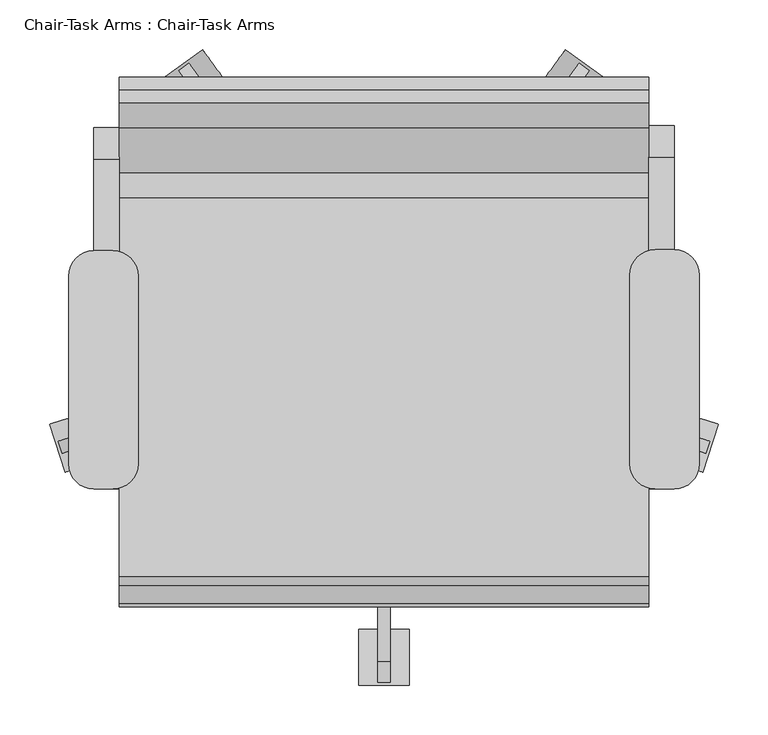
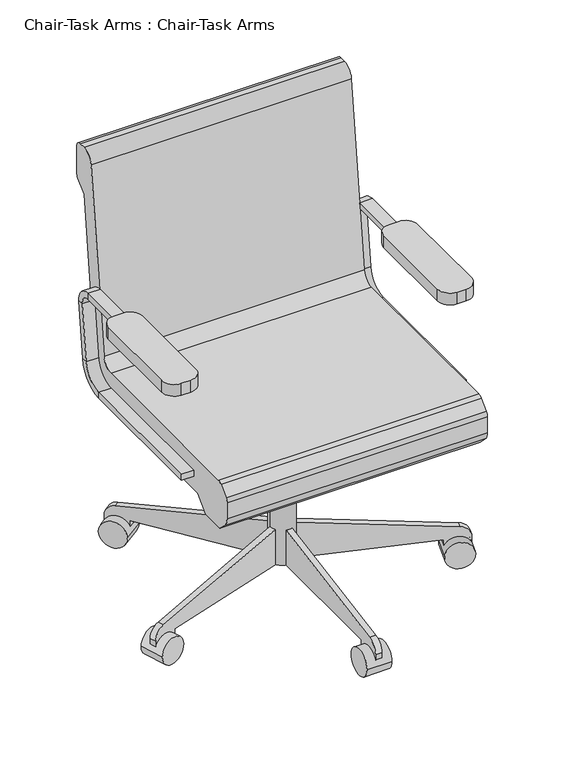
"""IFC4 building model written with IfcOpenShell, lengths in millimetres: furniture geometry, Chair-Task Arms : Chair-Task Arms."""

from ifc_helpers import new_model, si_unit, point, frame, frame_2d, origin, place, context, project, spatial, polyline, circle_curve, trimmed, segment, composite_curve, outline, extrude, source, transform, mapped, element, save
from ifc_brep_helpers import plane_surface, cylinder_surface, revolved_surface, advanced_brep


def chair_task_arms_chair_task_arms_3c69ee15(model_context):
    return source(origin(), model_context, "Body", "SolidModel", [
        extrude(outline(composite_curve([segment(trimmed(circle_curve(frame_2d((433.0908197, 48.8028048)), 25.4), [point((433.0908197, 74.2028048))], [point((458.4908197, 48.8028048))], False, "CARTESIAN"), True, "CONTINUOUS"), segment(polyline([(458.4908197, 48.8028048), (458.4908197, -141.6319091)]), True, "CONTINUOUS"), segment(trimmed(circle_curve(frame_2d((433.0908197, -141.6319091)), 25.4), [point((458.4908197, -141.6319091))], [point((433.0908197, -167.0319091))], False, "CARTESIAN"), True, "CONTINUOUS"), segment(polyline([(433.0908197, -167.0319091), (414.0408197, -167.0319091)]), True, "CONTINUOUS"), segment(trimmed(circle_curve(frame_2d((414.0408197, -141.6319091)), 25.4), [point((414.0408197, -167.0319091))], [point((388.6408197, -141.6319091))], False, "CARTESIAN"), True, "CONTINUOUS"), segment(polyline([(388.6408197, -141.6319091), (388.6408197, 48.8028048)]), True, "CONTINUOUS"), segment(trimmed(circle_curve(frame_2d((414.0408197, 48.8028048)), 25.4), [point((388.6408197, 48.8028048))], [point((414.0408197, 74.2028048))], False, "CARTESIAN"), True, "CONTINUOUS"), segment(polyline([(414.0408197, 74.2028048), (433.0908197, 74.2028048)]), True, "CONTINUOUS")], self_intersect=False)), frame((0.0, 0.0, 596.9), z_axis=(0.0, 0.0, 1.0), x_axis=(1.0, 0.0, 0.0)), (0.0, 0.0, 1.0), 25.4),
        extrude(outline(composite_curve([segment(trimmed(circle_curve(frame_2d((-132.0591803, 47.7575984)), 25.4), [point((-132.0591803, 73.1575984))], [point((-106.6591803, 47.7575984))], False, "CARTESIAN"), True, "CONTINUOUS"), segment(polyline([(-106.6591803, 47.7575984), (-106.6591803, -141.6319091)]), True, "CONTINUOUS"), segment(trimmed(circle_curve(frame_2d((-132.0591803, -141.6319091)), 25.4), [point((-106.6591803, -141.6319091))], [point((-132.0591803, -167.0319091))], False, "CARTESIAN"), True, "CONTINUOUS"), segment(polyline([(-132.0591803, -167.0319091), (-151.1091803, -167.0319091)]), True, "CONTINUOUS"), segment(trimmed(circle_curve(frame_2d((-151.1091803, -141.6319091)), 25.4), [point((-151.1091803, -167.0319091))], [point((-176.5091803, -141.6319091))], False, "CARTESIAN"), True, "CONTINUOUS"), segment(polyline([(-176.5091803, -141.6319091), (-176.5091803, 47.7575984)]), True, "CONTINUOUS"), segment(trimmed(circle_curve(frame_2d((-151.1091803, 47.7575984)), 25.4), [point((-176.5091803, 47.7575984))], [point((-151.1091803, 73.1575984))], False, "CARTESIAN"), True, "CONTINUOUS"), segment(polyline([(-151.1091803, 73.1575984), (-132.0591803, 73.1575984)]), True, "CONTINUOUS")], self_intersect=False)), frame((0.0, 0.0, 596.9), z_axis=(0.0, 0.0, 1.0), x_axis=(1.0, 0.0, 0.0)), (0.0, 0.0, 1.0), 25.4),
        advanced_brep(
        [(-151.1091803, -167.0319091, 412.75), (-125.7091803, -167.0319091, 412.75), (-125.7091803, -167.0319091, 425.45), (-151.1091803, -167.0319091, 425.45), (-151.1091803, 126.2388651, 425.45), (-151.1091803, 126.2388651, 412.75), (-125.7091803, 126.2388651, 425.45), (-125.7091803, 126.2388651, 412.75), (-151.1091803, 170.3844094, 464.7064065), (-151.1091803, 182.9974221, 463.2225227), (-125.7091803, 170.3844094, 464.7064065), (-125.7091803, 182.9974221, 463.2225227), (-151.1091803, 184.1806174, 581.9741742), (-151.1091803, 196.7936301, 580.4902904), (-125.7091803, 184.1806174, 581.9741742), (-125.7091803, 196.7936301, 580.4902904), (-151.1091803, 165.2610984, 603.25), (-151.1091803, 165.2610984, 615.95), (-125.7091803, 165.2610984, 603.25), (-125.7091803, 165.2610984, 615.95), (-151.1091803, -18.9459016, 615.95), (-151.1091803, -18.9459016, 603.25), (-125.7091803, -18.9459016, 603.25), (-125.7091803, -18.9459016, 615.95)],
        [
            (0, 1),
            (1, 2),
            (2, 3),
            (3, 0),
            (3, 4),
            (4, 5),
            (5, 0),
            (2, 6),
            (6, 4),
            (1, 7),
            (7, 6),
            (5, 7),
            (8, 9),
            (9, 5, circle_curve(frame((-151.1091803, 126.2388651, 469.9), z_axis=(-1.0, 0.0, 0.0), x_axis=(0.0, 0.0, -1.0)), 57.15)),
            (4, 8, circle_curve(frame((-151.1091803, 126.2388651, 469.9), z_axis=(1.0, 0.0, 0.0), x_axis=(0.0, 0.0, -1.0)), 44.45)),
            (10, 8),
            (6, 10, circle_curve(frame((-125.7091803, 126.2388651, 469.9), z_axis=(1.0, 0.0, 0.0), x_axis=(0.0, 0.0, -1.0)), 44.45)),
            (11, 10),
            (7, 11, circle_curve(frame((-125.7091803, 126.2388651, 469.9), z_axis=(1.0, 0.0, 0.0), x_axis=(0.0, 0.0, -1.0)), 57.15)),
            (9, 11),
            (8, 12),
            (12, 13),
            (13, 9),
            (10, 14),
            (14, 12),
            (11, 15),
            (15, 14),
            (13, 15),
            (16, 17),
            (17, 13, circle_curve(frame((-151.1091803, 165.2610984, 584.2), z_axis=(-1.0, 0.0, 0.0), x_axis=(0.0, 0.9931506043228768, -0.11684124756739202)), 31.75)),
            (12, 16, circle_curve(frame((-151.1091803, 165.2610984, 584.2), z_axis=(1.0, 0.0, 0.0), x_axis=(0.0, 0.9931506043228768, -0.11684124756739202)), 19.05)),
            (18, 16),
            (14, 18, circle_curve(frame((-125.7091803, 165.2610984, 584.2), z_axis=(1.0, 0.0, 0.0), x_axis=(0.0, 0.9931506043228768, -0.11684124756739202)), 19.05)),
            (19, 18),
            (15, 19, circle_curve(frame((-125.7091803, 165.2610984, 584.2), z_axis=(1.0, 0.0, 0.0), x_axis=(0.0, 0.9931506043228768, -0.11684124756739202)), 31.75)),
            (17, 19),
            (20, 21),
            (21, 22),
            (22, 23),
            (23, 20),
            (16, 21),
            (20, 17),
            (18, 22),
            (19, 23),
        ],
        [
            plane_surface(frame((-152.608212, -167.0319091, 419.1), z_axis=(0.0, -1.0, 0.0), x_axis=(0.0, 0.0, -1.0))),
            plane_surface(frame((-151.1091803, -167.0319091, 412.75), z_axis=(-1.0, 0.0, 0.0), x_axis=(0.0, 1.0, 0.0))),
            plane_surface(frame((-151.1091803, -167.0319091, 425.45), z_axis=(0.0, 0.0, 1.0), x_axis=(0.0, 1.0, 0.0))),
            plane_surface(frame((-125.7091803, -167.0319091, 425.45), z_axis=(1.0, 0.0, 0.0), x_axis=(0.0, 1.0, 0.0))),
            plane_surface(frame((-125.7091803, -167.0319091, 412.75), z_axis=(0.0, 0.0, -1.0), x_axis=(0.0, 1.0, 0.0))),
            plane_surface(frame((-151.1091803, 126.2388651, 469.9), z_axis=(-1.0, 0.0, 0.0), x_axis=(0.0, 0.0, -1.0))),
            revolved_surface(polyline([(-151.1091803, 126.2388651, 425.45), (-125.7091803, 126.2388651, 425.45)]), (-138.4091803, 126.2388651, 469.9), (-1.0, 0.0, 0.0)),
            plane_surface(frame((-125.7091803, 126.2388651, 469.9), z_axis=(1.0, 0.0, 0.0), x_axis=(0.0, 0.0, -1.0))),
            cylinder_surface(frame((-138.4091803, 126.2388651, 469.9), z_axis=(-1.0, 0.0, 0.0), x_axis=(0.0, 0.0, -1.0)), 57.15),
            plane_surface(frame((-151.1091803, 182.9974221, 463.2225227), z_axis=(-1.0, 0.0, 0.0), x_axis=(0.0, 0.1168412475673856, 0.9931506043228776))),
            plane_surface(frame((-151.1091803, 170.3844094, 464.7064065), z_axis=(0.0, -0.9931506043228776, 0.1168412475673856), x_axis=(0.0, 0.1168412475673856, 0.9931506043228776))),
            plane_surface(frame((-125.7091803, 170.3844094, 464.7064065), z_axis=(1.0, 0.0, 0.0), x_axis=(0.0, 0.1168412475673856, 0.9931506043228776))),
            plane_surface(frame((-125.7091803, 182.9974221, 463.2225227), z_axis=(0.0, 0.9931506043228776, -0.1168412475673856), x_axis=(0.0, 0.1168412475673856, 0.9931506043228776))),
            plane_surface(frame((-151.1091803, 165.2610984, 584.2), z_axis=(-1.0, 0.0, 0.0), x_axis=(0.0, 0.9931506043228768, -0.11684124756739202))),
            revolved_surface(polyline([(-151.1091803, 184.1806174123508, 581.9741742338413), (-125.7091803, 184.1806174123508, 581.9741742338413)]), (-138.4091803, 165.2610984, 584.2), (-1.0, 0.0, 0.0)),
            plane_surface(frame((-125.7091803, 165.2610984, 584.2), z_axis=(1.0, 0.0, 0.0), x_axis=(0.0, 0.9931506043228768, -0.11684124756739202))),
            cylinder_surface(frame((-138.4091803, 165.2610984, 584.2), z_axis=(-1.0, 0.0, 0.0), x_axis=(0.0, 0.9931506043228768, -0.11684124756739202)), 31.75),
            plane_surface(frame((-152.608212, -18.9459016, 609.6), z_axis=(0.0, -1.0, 0.0), x_axis=(0.0, 0.0, 1.0))),
            plane_surface(frame((-151.1091803, 165.2610984, 615.95), z_axis=(-1.0, 0.0, 0.0), x_axis=(0.0, -1.0, 0.0))),
            plane_surface(frame((-151.1091803, 165.2610984, 603.25), z_axis=(0.0, 0.0, -1.0), x_axis=(0.0, -1.0, 0.0))),
            plane_surface(frame((-125.7091803, 165.2610984, 603.25), z_axis=(1.0, 0.0, 0.0), x_axis=(0.0, -1.0, 0.0))),
            plane_surface(frame((-125.7091803, 165.2610984, 615.95), z_axis=(0.0, 0.0, 1.0), x_axis=(0.0, -1.0, 0.0))),
        ],
        [
            (0, [[1, 2, 3, 4]]),
            (1, [[5, 6, 7, -4]]),
            (2, [[8, 9, -5, -3]]),
            (3, [[10, 11, -8, -2]]),
            (4, [[-7, 12, -10, -1]]),
            (5, [[13, 14, -6, 15]]),
            (6, [[16, -15, -9, 17]]),
            (7, [[18, -17, -11, 19]]),
            (8, [[20, -19, -12, -14]]),
            (9, [[21, 22, 23, -13]]),
            (10, [[24, 25, -21, -16]]),
            (11, [[26, 27, -24, -18]]),
            (12, [[-23, 28, -26, -20]]),
            (13, [[29, 30, -22, 31]]),
            (14, [[32, -31, -25, 33]]),
            (15, [[34, -33, -27, 35]]),
            (16, [[36, -35, -28, -30]]),
            (17, [[37, 38, 39, 40]]),
            (18, [[41, -37, 42, -29]]),
            (19, [[43, -38, -41, -32]]),
            (20, [[44, -39, -43, -34]]),
            (21, [[-42, -40, -44, -36]]),
        ],
    ),
        advanced_brep(
        [(433.0908197, -167.0319091, 425.45), (407.6908197, -167.0319091, 425.45), (407.6908197, -167.0319091, 412.75), (433.0908197, -167.0319091, 412.75), (433.0908197, 128.329278, 412.75), (433.0908197, 128.329278, 425.45), (407.6908197, 128.329278, 412.75), (407.6908197, 128.329278, 425.45), (433.0908197, 185.0878351, 463.2225227), (433.0908197, 172.4748224, 464.7064065), (407.6908197, 185.0878351, 463.2225227), (407.6908197, 172.4748224, 464.7064065), (433.0908197, 198.884043, 580.4902904), (433.0908197, 186.2710303, 581.9741742), (407.6908197, 198.884043, 580.4902904), (407.6908197, 186.2710303, 581.9741742), (433.0908197, 167.3515113, 615.95), (433.0908197, 167.3515113, 603.25), (407.6908197, 167.3515113, 615.95), (407.6908197, 167.3515113, 603.25), (433.0908197, -18.9459016, 603.25), (433.0908197, -18.9459016, 615.95), (407.6908197, -18.9459016, 615.95), (407.6908197, -18.9459016, 603.25)],
        [
            (0, 1),
            (1, 2),
            (2, 3),
            (3, 0),
            (3, 4),
            (4, 5),
            (5, 0),
            (2, 6),
            (6, 4),
            (1, 7),
            (7, 6),
            (5, 7),
            (8, 9),
            (9, 5, circle_curve(frame((433.0908197, 128.329278, 469.9), z_axis=(-1.0, 0.0, 0.0), x_axis=(0.0, 0.0, -1.0)), 44.45)),
            (4, 8, circle_curve(frame((433.0908197, 128.329278, 469.9), z_axis=(1.0, 0.0, 0.0), x_axis=(0.0, 0.0, -1.0)), 57.15)),
            (10, 8),
            (6, 10, circle_curve(frame((407.6908197, 128.329278, 469.9), z_axis=(1.0, 0.0, 0.0), x_axis=(0.0, 0.0, -1.0)), 57.15)),
            (11, 10),
            (7, 11, circle_curve(frame((407.6908197, 128.329278, 469.9), z_axis=(1.0, 0.0, 0.0), x_axis=(0.0, 0.0, -1.0)), 44.45)),
            (9, 11),
            (8, 12),
            (12, 13),
            (13, 9),
            (10, 14),
            (14, 12),
            (11, 15),
            (15, 14),
            (13, 15),
            (16, 17),
            (17, 13, circle_curve(frame((433.0908197, 167.3515113, 584.2), z_axis=(-1.0, 0.0, 0.0), x_axis=(0.0, 0.9931506043228767, -0.1168412475673929)), 19.05)),
            (12, 16, circle_curve(frame((433.0908197, 167.3515113, 584.2), z_axis=(1.0, 0.0, 0.0), x_axis=(0.0, 0.9931506043228767, -0.1168412475673929)), 31.75)),
            (18, 16),
            (14, 18, circle_curve(frame((407.6908197, 167.3515113, 584.2), z_axis=(1.0, 0.0, 0.0), x_axis=(0.0, 0.9931506043228767, -0.1168412475673929)), 31.75)),
            (19, 18),
            (15, 19, circle_curve(frame((407.6908197, 167.3515113, 584.2), z_axis=(1.0, 0.0, 0.0), x_axis=(0.0, 0.9931506043228767, -0.1168412475673929)), 19.05)),
            (17, 19),
            (20, 21),
            (21, 22),
            (22, 23),
            (23, 20),
            (16, 21),
            (20, 17),
            (18, 22),
            (19, 23),
        ],
        [
            plane_surface(frame((406.191788, -167.0319091, 419.1), z_axis=(0.0, -1.0, 0.0), x_axis=(0.0, 0.0, -1.0))),
            plane_surface(frame((433.0908197, -167.0319091, 425.45), z_axis=(1.0, 0.0, 0.0), x_axis=(0.0, 1.0, 0.0))),
            plane_surface(frame((433.0908197, -167.0319091, 412.75), z_axis=(0.0, 0.0, -1.0), x_axis=(0.0, 1.0, 0.0))),
            plane_surface(frame((407.6908197, -167.0319091, 412.75), z_axis=(-1.0, 0.0, 0.0), x_axis=(0.0, 1.0, 0.0))),
            plane_surface(frame((407.6908197, -167.0319091, 425.45), z_axis=(0.0, 0.0, 1.0), x_axis=(0.0, 1.0, 0.0))),
            plane_surface(frame((433.0908197, 128.329278, 469.9), z_axis=(1.0, 0.0, 0.0), x_axis=(0.0, 0.0, -1.0))),
            cylinder_surface(frame((420.3908197, 128.329278, 469.9), z_axis=(-1.0, 0.0, 0.0), x_axis=(0.0, 0.0, -1.0)), 57.15),
            plane_surface(frame((407.6908197, 128.329278, 469.9), z_axis=(-1.0, 0.0, 0.0), x_axis=(0.0, 0.0, -1.0))),
            revolved_surface(polyline([(407.6908197, 128.329278, 425.45), (433.0908197, 128.329278, 425.45)]), (420.3908197, 128.329278, 469.9), (-1.0, 0.0, 0.0)),
            plane_surface(frame((433.0908197, 172.4748224, 464.7064065), z_axis=(1.0, 0.0, 0.0), x_axis=(0.0, 0.11684124756738626, 0.9931506043228775))),
            plane_surface(frame((433.0908197, 185.0878351, 463.2225227), z_axis=(0.0, 0.9931506043228775, -0.11684124756738655), x_axis=(0.0, 0.11684124756738655, 0.9931506043228775))),
            plane_surface(frame((407.6908197, 185.0878351, 463.2225227), z_axis=(-1.0, 0.0, 0.0), x_axis=(0.0, 0.11684124756738626, 0.9931506043228775))),
            plane_surface(frame((407.6908197, 172.4748224, 464.7064065), z_axis=(0.0, -0.9931506043228775, 0.11684124756738626), x_axis=(0.0, 0.11684124756738626, 0.9931506043228775))),
            plane_surface(frame((433.0908197, 167.3515113, 584.2), z_axis=(1.0, 0.0, 0.0), x_axis=(0.0, 0.9931506043228767, -0.1168412475673929))),
            cylinder_surface(frame((420.3908197, 167.3515113, 584.2), z_axis=(-1.0, 0.0, 0.0), x_axis=(0.0, 0.9931506043228767, -0.1168412475673929)), 31.75),
            plane_surface(frame((407.6908197, 167.3515113, 584.2), z_axis=(-1.0, 0.0, 0.0), x_axis=(0.0, 0.9931506043228767, -0.1168412475673929))),
            revolved_surface(polyline([(407.6908197, 186.2710303123508, 581.9741742338412), (433.0908197, 186.2710303123508, 581.9741742338412)]), (420.3908197, 167.3515113, 584.2), (-1.0, 0.0, 0.0)),
            plane_surface(frame((406.191788, -18.9459016, 609.6), z_axis=(0.0, -1.0, 0.0), x_axis=(0.0, 0.0, 1.0))),
            plane_surface(frame((433.0908197, 167.3515113, 603.25), z_axis=(1.0, 0.0, 0.0), x_axis=(0.0, -1.0, 0.0))),
            plane_surface(frame((433.0908197, 167.3515113, 615.95), z_axis=(0.0, 0.0, 1.0), x_axis=(0.0, -1.0, 0.0))),
            plane_surface(frame((407.6908197, 167.3515113, 615.95), z_axis=(-1.0, 0.0, 0.0), x_axis=(0.0, -1.0, 0.0))),
            plane_surface(frame((407.6908197, 167.3515113, 603.25), z_axis=(0.0, 0.0, -1.0), x_axis=(0.0, -1.0, 0.0))),
        ],
        [
            (0, [[1, 2, 3, 4]]),
            (1, [[5, 6, 7, -4]]),
            (2, [[8, 9, -5, -3]]),
            (3, [[10, 11, -8, -2]]),
            (4, [[-7, 12, -10, -1]]),
            (5, [[13, 14, -6, 15]]),
            (6, [[16, -15, -9, 17]]),
            (7, [[18, -17, -11, 19]]),
            (8, [[20, -19, -12, -14]]),
            (9, [[21, 22, 23, -13]]),
            (10, [[24, 25, -21, -16]]),
            (11, [[26, 27, -24, -18]]),
            (12, [[-23, 28, -26, -20]]),
            (13, [[29, 30, -22, 31]]),
            (14, [[32, -31, -25, 33]]),
            (15, [[34, -33, -27, 35]]),
            (16, [[36, -35, -28, -30]]),
            (17, [[37, 38, 39, 40]]),
            (18, [[41, -37, 42, -29]]),
            (19, [[43, -38, -41, -32]]),
            (20, [[44, -39, -43, -34]]),
            (21, [[-42, -40, -44, -36]]),
        ],
    ),
        extrude(outline(composite_curve([segment(trimmed(circle_curve(frame_2d((140.9908197, -18.9459016)), 25.4), [point((115.5908197, -18.9459016))], [point((166.3908197, -18.9459016))], False, "CARTESIAN"), True, "CONTINUOUS"), segment(trimmed(circle_curve(frame_2d((140.9908197, -18.9459016)), 25.4), [point((166.3908197, -18.9459016))], [point((115.5908197, -18.9459016))], False, "CARTESIAN"), True, "CONTINUOUS")], self_intersect=False)), frame((0.0, 0.0, 53.5835944), z_axis=(0.0, 0.0, 1.0), x_axis=(1.0, 0.0, 0.0)), (0.0, 0.0, 1.0), 330.5914056),
        extrude(outline(composite_curve([segment(trimmed(circle_curve(frame_2d((0.0, 28.2002728)), 28.2002727), [point((0.0, 56.4005455))], [point((0.0, 0.0))], False, "CARTESIAN"), True, "CONTINUOUS"), segment(trimmed(circle_curve(frame_2d((0.0, 28.2002728)), 28.2002727), [point((0.0, 0.0))], [point((0.0, 56.4005455))], False, "CARTESIAN"), True, "CONTINUOUS")], self_intersect=False)), frame((461.9222851, -149.9299964, 28.1835944), z_axis=(0.3090169943749423, 0.9510565162951553, 0.0), x_axis=(0.0, 0.0, -1.0)), (0.0, 0.0, 1.0), 50.8),
        extrude(outline(composite_curve([segment(polyline([(25.4, 0.0), (0.0, 0.0), (0.0, 50.8), (24.303053, 50.8)]), True, "CONTINUOUS"), segment(trimmed(circle_curve(frame_2d((24.303053, 25.4)), 25.4), [point((24.303053, 50.8))], [point((49.3171699, 29.8106636))], False, "CARTESIAN"), True, "CONTINUOUS"), segment(polyline([(49.3171699, 29.8106636), (101.6, -266.7), (101.6, -292.1), (25.4, -292.1), (25.4, 0.0)]), True, "CONTINUOUS")], self_intersect=False)), frame((416.8321702, -115.2489746, 28.1835944), z_axis=(0.3090169943749423, 0.9510565162951553, 0.0), x_axis=(0.0, 0.0, 1.0)), (0.0, 0.0, 1.0), 12.7),
        extrude(outline(composite_curve([segment(trimmed(circle_curve(frame_2d((0.0, 28.2002726)), 28.2002727), [point((0.0, 56.4005454))], [point((0.0, 0.0))], False, "CARTESIAN"), True, "CONTINUOUS"), segment(trimmed(circle_curve(frame_2d((0.0, 28.2002726)), 28.2002727), [point((0.0, 0.0))], [point((0.0, 56.4005454))], False, "CARTESIAN"), True, "CONTINUOUS")], self_intersect=False)), frame((364.7373733, 245.8017485, 28.1835944), z_axis=(-0.8090169943749499, 0.5877852522924699, 0.0), x_axis=(0.0, 0.0, -1.0)), (0.0, 0.0, 1.0), 50.8),
        extrude(outline(composite_curve([segment(polyline([(25.4, 0.0), (0.0, 0.0), (0.0, 50.8), (24.303053, 50.8)]), True, "CONTINUOUS"), segment(trimmed(circle_curve(frame_2d((24.303053, 25.3999999)), 25.4), [point((24.303053, 50.8))], [point((49.3171699, 29.8106637))], False, "CARTESIAN"), True, "CONTINUOUS"), segment(polyline([(49.3171699, 29.8106637), (101.6, -266.7), (101.6, -292.1), (25.4, -292.1), (25.4, 0.0)]), True, "CONTINUOUS")], self_intersect=False)), frame((317.8201498, 213.6355261, 28.1835944), z_axis=(-0.8090169943749499, 0.5877852522924699, 0.0), x_axis=(0.0, 0.0, 1.0)), (0.0, 0.0, 1.0), 12.7),
        extrude(outline(composite_curve([segment(trimmed(circle_curve(frame_2d((0.0, 28.2002726)), 28.2002727), [point((0.0, 56.4005454))], [point((0.0, 0.0))], False, "CARTESIAN"), True, "CONTINUOUS"), segment(trimmed(circle_curve(frame_2d((0.0, 28.2002726)), 28.2002727), [point((0.0, 0.0))], [point((0.0, 56.4005454))], False, "CARTESIAN"), True, "CONTINUOUS")], self_intersect=False)), frame((-82.755734, 245.8017485, 28.1835944), z_axis=(0.8090169943749458, 0.5877852522924754, 0.0), x_axis=(0.0, 0.0, 1.0)), (0.0, 0.0, 1.0), 50.8),
        extrude(outline(composite_curve([segment(polyline([(-25.4, 0.0), (-25.4, -292.1), (-101.6, -292.1), (-101.6, -266.6999999), (-49.3171699, 29.8106637)]), True, "CONTINUOUS"), segment(trimmed(circle_curve(frame_2d((-24.303053, 25.3999999)), 25.4), [point((-49.3171699, 29.8106637))], [point((-24.303053, 50.8))], False, "CARTESIAN"), True, "CONTINUOUS"), segment(polyline([(-24.303053, 50.8), (0.0, 50.8), (0.0, 0.0), (-25.4, 0.0)]), True, "CONTINUOUS")], self_intersect=False)), frame((-35.8385104, 213.6355261, 28.1835944), z_axis=(0.8090169943749459, 0.5877852522924754, 0.0), x_axis=(0.0, 0.0, -1.0)), (0.0, 0.0, 1.0), 12.7),
        extrude(outline(composite_curve([segment(trimmed(circle_curve(frame_2d((0.0, 28.2002727)), 28.2002727), [point((0.0, 56.4005454))], [point((0.0, 0.0))], False, "CARTESIAN"), True, "CONTINUOUS"), segment(trimmed(circle_curve(frame_2d((0.0, 28.2002727)), 28.2002727), [point((0.0, 0.0))], [point((0.0, 56.4005454))], False, "CARTESIAN"), True, "CONTINUOUS")], self_intersect=False)), frame((-179.9406457, -149.9299964, 28.1835944), z_axis=(-0.3090169943749487, 0.9510565162951532, 0.0), x_axis=(0.0, 0.0, 1.0)), (0.0, 0.0, 1.0), 50.8),
        extrude(outline(composite_curve([segment(polyline([(-25.4, 0.0), (-25.4, -292.1), (-101.6, -292.1), (-101.6, -266.7), (-49.3171699, 29.8106637)]), True, "CONTINUOUS"), segment(trimmed(circle_curve(frame_2d((-24.303053, 25.4)), 25.4), [point((-49.3171699, 29.8106637))], [point((-24.303053, 50.8000001))], False, "CARTESIAN"), True, "CONTINUOUS"), segment(polyline([(-24.303053, 50.8000001), (0.0, 50.8000001), (0.0, 0.0), (-25.4, 0.0)]), True, "CONTINUOUS")], self_intersect=False)), frame((-134.8505308, -115.2489746, 28.1835944), z_axis=(-0.3090169943749487, 0.9510565162951532, 0.0), x_axis=(0.0, 0.0, -1.0)), (0.0, 0.0, 1.0), 12.7),
        extrude(outline(composite_curve([segment(trimmed(circle_curve(frame_2d((-336.4459016, 28.1835944)), 28.2002727), [point((-308.2456289, 28.1835944))], [point((-364.6461744, 28.1835944))], False, "CARTESIAN"), True, "CONTINUOUS"), segment(trimmed(circle_curve(frame_2d((-336.4459016, 28.1835944)), 28.2002727), [point((-364.6461744, 28.1835944))], [point((-308.2456289, 28.1835944))], False, "CARTESIAN"), True, "CONTINUOUS")], self_intersect=False)), frame((115.5908197, 0.0, 0.0), z_axis=(1.0, 0.0, 0.0), x_axis=(0.0, 1.0, 0.0)), (0.0, 0.0, 1.0), 50.8),
        extrude(outline(composite_curve([segment(polyline([(-311.0459016, 53.5835944), (-311.0459016, 28.1835944), (-361.8459016, 28.1835944), (-361.8459016, 52.4866474)]), True, "CONTINUOUS"), segment(trimmed(circle_curve(frame_2d((-336.4459016, 52.4866474)), 25.4), [point((-361.8459016, 52.4866474))], [point((-340.8565654, 77.5007643))], False, "CARTESIAN"), True, "CONTINUOUS"), segment(polyline([(-340.8565654, 77.5007643), (-44.3459016, 129.7835944), (-18.9459016, 129.7835944), (-18.9459016, 53.5835944), (-311.0459016, 53.5835944)]), True, "CONTINUOUS")], self_intersect=False)), frame((134.6408197, 0.0, 0.0), z_axis=(1.0, 0.0, 0.0), x_axis=(0.0, 1.0, 0.0)), (0.0, 0.0, 1.0), 12.7),
        extrude(outline(polyline([(-69.7459016, 383.7835944), (19.1540984, 383.7835944), (19.1540984, 283.0954134), (-18.9459016, 283.0954134), (-69.7459016, 371.0835944), (-69.7459016, 383.7835944)])), frame((90.1908197, 0.0, 0.0), z_axis=(1.0, 0.0, 0.0), x_axis=(0.0, 1.0, 0.0)), (0.0, 0.0, 1.0), 101.6),
        extrude(outline(composite_curve([segment(trimmed(circle_curve(frame_2d((126.2050455, 482.6)), 25.4), [point((126.2050455, 457.2))], [point((151.4310708, 479.6322323))], True, "CARTESIAN"), True, "CONTINUOUS"), segment(polyline([(151.4310708, 479.6322323), (196.9528985, 866.5677677)]), True, "CONTINUOUS"), segment(trimmed(circle_curve(frame_2d((222.1789239, 863.6)), 25.4), [point((196.9528985, 866.5677677))], [point((222.1789239, 889.0))], False, "CARTESIAN"), True, "CONTINUOUS"), segment(polyline([(222.1789239, 889.0), (235.0540984, 889.0)]), True, "CONTINUOUS"), segment(trimmed(circle_curve(frame_2d((235.0540984, 876.3)), 12.7), [point((235.0540984, 889.0))], [point((247.7540984, 876.3))], False, "CARTESIAN"), True, "CONTINUOUS"), segment(polyline([(247.7540984, 876.3), (247.7540984, 818.0605122)]), True, "CONTINUOUS"), segment(trimmed(circle_curve(frame_2d((235.0540984, 818.0605122)), 12.7), [point((247.7540984, 818.0605122))], [point((244.0343545, 809.0802561))], False, "CARTESIAN"), True, "CONTINUOUS"), segment(polyline([(244.0343545, 809.0802561), (222.3540984, 787.4), (182.7870738, 451.0802913)]), True, "CONTINUOUS"), segment(trimmed(circle_curve(frame_2d((107.1089978, 459.9835944)), 76.2), [point((182.7870738, 451.0802913))], [point((107.1089978, 383.7835944))], False, "CARTESIAN"), True, "CONTINUOUS"), segment(polyline([(107.1089978, 383.7835944), (-181.0744602, 383.7835944), (-209.4470284, 355.6), (-260.2470284, 355.6), (-278.2663256, 373.7401184)]), True, "CONTINUOUS"), segment(trimmed(circle_curve(frame_2d((-260.2459016, 391.6405184)), 25.4), [point((-278.2663256, 373.7401184))], [point((-285.6459016, 391.6405184))], False, "CARTESIAN"), True, "CONTINUOUS"), segment(polyline([(-285.6459016, 391.6405184), (-285.6459016, 426.6837879)]), True, "CONTINUOUS"), segment(trimmed(circle_curve(frame_2d((-272.9459016, 426.6837879)), 12.7), [point((-285.6459016, 426.6837879))], [point((-281.8961016, 435.6939999))], False, "CARTESIAN"), True, "CONTINUOUS"), segment(polyline([(-281.8961016, 435.6939999), (-263.9604301, 453.510212)]), True, "CONTINUOUS"), segment(trimmed(circle_curve(frame_2d((-255.0102301, 444.5)), 12.7), [point((-263.9604301, 453.510212))], [point((-255.0102301, 457.2))], False, "CARTESIAN"), True, "CONTINUOUS"), segment(polyline([(-255.0102301, 457.2), (126.2050455, 457.2)]), True, "CONTINUOUS")], self_intersect=False)), frame((-125.7091803, 0.0, 0.0), z_axis=(1.0, 0.0, 0.0), x_axis=(0.0, 1.0, 0.0)), (0.0, 0.0, 1.0), 533.4),
    ])


if __name__ == "__main__":
    model = new_model("IFC4")
    model_context = context("Model", 3, world=origin())
    ifc_project = project(units=[si_unit("LENGTHUNIT", "METRE", prefix="MILLI")], contexts=[model_context])
    site = spatial("IfcSite", under=ifc_project)
    building = spatial("IfcBuilding", under=site)
    placement = place(None, origin())
    chair_task_arms_chair_task_arms_shape = chair_task_arms_chair_task_arms_3c69ee15(model_context)
    element("IfcFurniture", 1, ObjectType="Chair-Task Arms : Chair-Task Arms", at=placement, inside=building, context=model_context, shape_type="MappedRepresentation", body=[
        mapped(chair_task_arms_chair_task_arms_shape, transform((0.0, 0.0, 0.0), x_axis=(1.0, 0.0, 0.0), y_axis=(0.0, 1.0, 0.0), z_axis=(0.0, 0.0, 1.0))),
    ])
    save(model, "model.ifc")

# Revit data of these elements
# Type "Chair-Task Arms : Chair-Task Arms"
#   Assembly Code = "E2020200"
#   Base Material = Plastic, Opaque Black
#   Caster Material = Plastic, Opaque Black
#   Seat/Back Material = Textile - Slate Blue
#   Default Elevation = 0
# Element 1 (IfcFurniture, "Chair-Task Arms : Chair-Task Arms")
#   Materials on its faces: "Plastic, Opaque Black", "Textile - Slate Blue"
# Materials
#   "Plastic, Opaque Black": class "Plastic", colour RGB 0 0 0, transparency 0, Description = "Plastic, generic, opaque black", Cost = 0
#   "Textile - Slate Blue": class "Fabric", colour RGB 98 102 118, transparency 0
